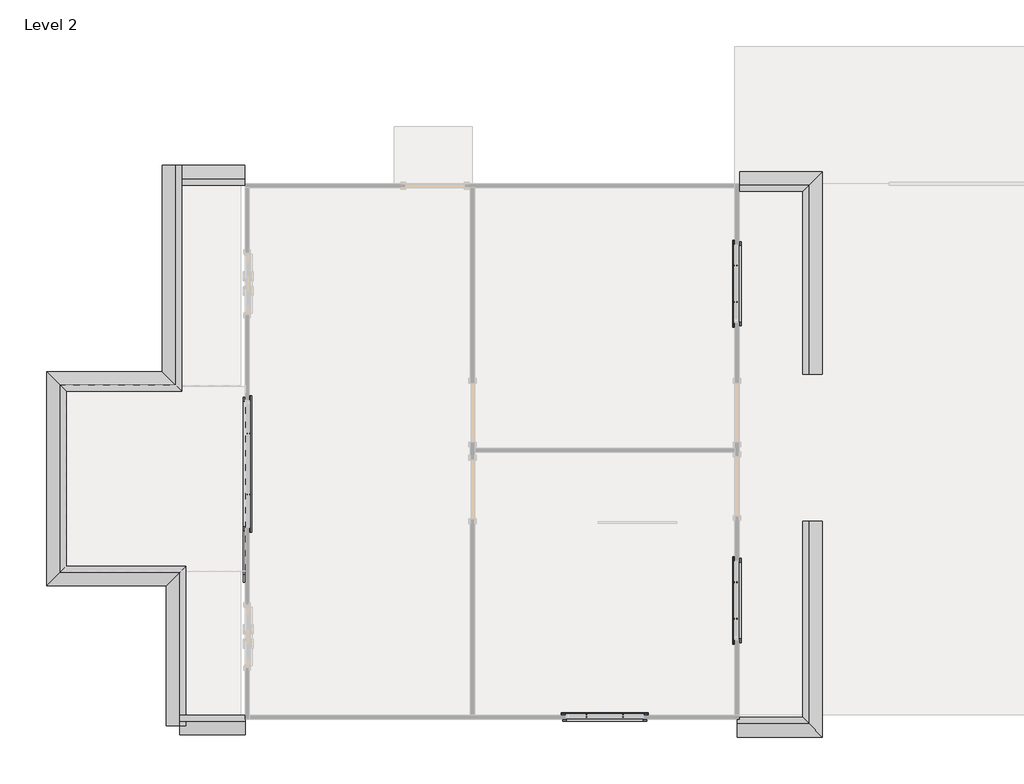
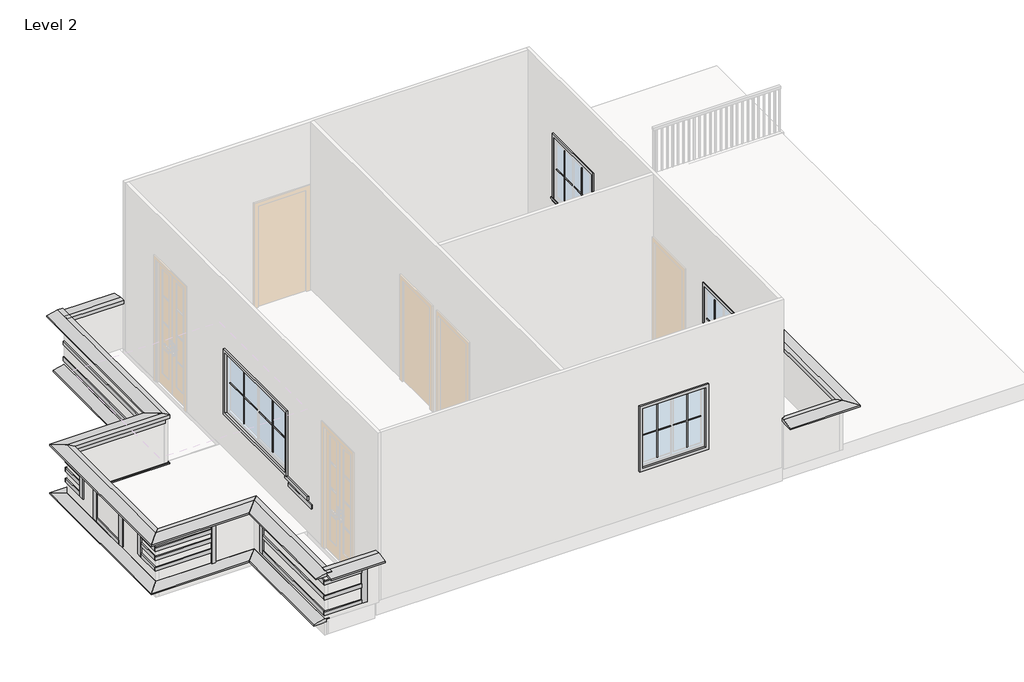
# One storey, part 2 of 2: 41 furniture elements, 34 proxies.
"""IFC4 building model written with IfcOpenShell, lengths in millimetres."""

import ifcopenshell
import ifcopenshell.guid

model = None  # the IFC model being written
_history = None  # IfcOwnerHistory: only IFC2X3 demands one
_inside = {}  # id of a spatial element -> (the spatial element, [elements in it])
_under = {}  # id of a project, library or spatial element -> (it, [spatial elements below it])
_declared = {}  # id of a project -> (the project, [libraries it declares])
_typed = {}  # id of a type object -> (the type object, [elements of that type])
_made_of = {}  # id of a material, layer set ... -> (it, [elements and type objects made of it])


def new_model(schema):
    """Start an empty IFC model of exactly this schema.

    Asked for "IFC4X3", IfcOpenShell would pick the latest addendum, in which some entities
    have other attributes; the version numbers below select the first issue.
    IFC2X3 requires an IfcOwnerHistory on every rooted entity: one is made here for all.
    """
    global model, _history
    if schema == "IFC4X3":
        model = ifcopenshell.file(schema_version=(4, 3, 0, 0))
    else:
        model = ifcopenshell.file(schema=schema)
    _inside.clear()
    _under.clear()
    _declared.clear()
    _typed.clear()
    _made_of.clear()
    _history = None
    if model.schema == "IFC2X3":
        org = make("IfcOrganization", Name="unknown")
        user = make(
            "IfcPersonAndOrganization",
            ThePerson=make("IfcPerson", FamilyName="unknown"),
            TheOrganization=org,
        )
        app = make(
            "IfcApplication",
            ApplicationDeveloper=org,
            Version="unknown",
            ApplicationFullName="unknown",
            ApplicationIdentifier="unknown",
        )
        _history = make(
            "IfcOwnerHistory",
            OwningUser=user,
            OwningApplication=app,
            ChangeAction="ADDED",
            CreationDate=0,
        )
    return model


def make(cls, **values):
    """One entity of the class cls with the attributes given. An attribute that is None is left unset."""
    return model.create_entity(
        cls, **{name: value for name, value in values.items() if value is not None}
    )


def rooted(cls, **values):
    """An entity with a GlobalId (a new one), such as an element, a storey or a relation."""
    return make(cls, GlobalId=ifcopenshell.guid.new(), OwnerHistory=_history, **values)


def si_unit(unit_type, name, prefix=None):
    """IfcSIUnit, for example si_unit("LENGTHUNIT", "METRE", prefix="MILLI")."""
    return make("IfcSIUnit", UnitType=unit_type, Prefix=prefix, Name=name)


def assignment(units):
    """IfcUnitAssignment: the units of a project."""
    return None if units is None else make("IfcUnitAssignment", Units=units)


def point(xyz):
    """IfcCartesianPoint."""
    return None if xyz is None else make("IfcCartesianPoint", Coordinates=xyz)


def direction(xyz):
    """IfcDirection."""
    return None if xyz is None else make("IfcDirection", DirectionRatios=xyz)


def frame(location, z_axis=None, x_axis=None):
    """IfcAxis2Placement3D, a coordinate frame: its origin and axes. An axis left out is left unset."""
    return make(
        "IfcAxis2Placement3D",
        Location=point(location),
        Axis=direction(z_axis),
        RefDirection=direction(x_axis),
    )


def origin():
    """The frame at (0, 0, 0) with its axes left unset."""
    return frame((0.0, 0.0, 0.0))


def origin_with_axes():
    """The frame at (0, 0, 0) with the z axis (0, 0, 1) and the x axis (1, 0, 0) written out."""
    return frame((0.0, 0.0, 0.0), z_axis=(0.0, 0.0, 1.0), x_axis=(1.0, 0.0, 0.0))


def place(relative_to, where):
    """IfcLocalPlacement: puts the frame where relative to a parent placement (None: the world)."""
    return make(
        "IfcLocalPlacement", PlacementRelTo=relative_to, RelativePlacement=where
    )


def context(
    kind, dimensions, precision=None, world=None, true_north=None, identifier=None
):
    """IfcGeometricRepresentationContext, for example the 3D "Model" context."""
    return make(
        "IfcGeometricRepresentationContext",
        ContextIdentifier=identifier,
        ContextType=kind,
        CoordinateSpaceDimension=dimensions,
        Precision=precision,
        WorldCoordinateSystem=world,
        TrueNorth=true_north,
    )


def project(units=None, contexts=None):
    """IfcProject with its units and contexts."""
    return rooted(
        "IfcProject",
        Name="project",
        RepresentationContexts=contexts,
        UnitsInContext=assignment(units),
    )


def spatial(cls, under=None, at=None, **own):
    """A site, building, storey or space (cls), placed at a placement, below another one or the project."""
    s = rooted(cls, ObjectPlacement=at, **own)
    if under is not None:
        _under.setdefault(under.id(), (under, []))[1].append(s)
    return s


def polyline(points):
    """IfcPolyline through the points."""
    return make("IfcPolyline", Points=[point(p) for p in points])


def outline(outer, holes=None, kind="AREA"):
    """IfcArbitraryClosedProfileDef: a profile drawn as a closed curve; with holes, ...WithVoids."""
    if holes is None:
        return make("IfcArbitraryClosedProfileDef", ProfileType=kind, OuterCurve=outer)
    return make(
        "IfcArbitraryProfileDefWithVoids",
        ProfileType=kind,
        OuterCurve=outer,
        InnerCurves=holes,
    )


def extrude(swept, where, along, depth):
    """IfcExtrudedAreaSolid: the profile swept, set in the frame where, extruded along a direction by depth."""
    return make(
        "IfcExtrudedAreaSolid",
        SweptArea=swept,
        Position=where,
        ExtrudedDirection=direction(along),
        Depth=depth,
    )


def faces_of(points, faces, orient=None, outer=None):
    """IfcFace entities. A face is a list of loops; a loop is a list of indices into points, from 0.

    orient and outer hold one flag for each loop. By default every Orientation is true, the
    first loop of a face is its IfcFaceOuterBound and the others are IfcFaceBound.
    """
    made = []
    for i, loops in enumerate(faces):
        bounds = []
        for j, loop in enumerate(loops):
            is_outer = j == 0 if outer is None else outer[i][j]
            bounds.append(
                make(
                    "IfcFaceOuterBound" if is_outer else "IfcFaceBound",
                    Bound=make("IfcPolyLoop", Polygon=[points[k] for k in loop]),
                    Orientation=True if orient is None else orient[i][j],
                )
            )
        made.append(make("IfcFace", Bounds=bounds))
    return made


def faceted_brep(points, faces, orient=None, outer=None, voids=None):
    """IfcFacetedBrep: a solid bounded by flat faces; with voids (closed shells), ...WithVoids."""
    shared = [point(p) for p in points]
    hull = make("IfcClosedShell", CfsFaces=faces_of(shared, faces, orient, outer))
    if voids is None:
        return make("IfcFacetedBrep", Outer=hull)
    return make(
        "IfcFacetedBrepWithVoids",
        Outer=hull,
        Voids=[
            make(cls, CfsFaces=faces_of(shared, fs, o, b)) for cls, fs, o, b in voids
        ],
    )


def shape(context_of_items, identifier, shape_type, items):
    """IfcShapeRepresentation: the items that make up one representation, for example the "Body"."""
    return make(
        "IfcShapeRepresentation",
        ContextOfItems=context_of_items,
        RepresentationIdentifier=identifier,
        RepresentationType=shape_type,
        Items=items,
    )


def source(mapping_origin, context_of_items, identifier, shape_type, items):
    """IfcRepresentationMap: a shape defined once, which mapped items show again and again."""
    return make(
        "IfcRepresentationMap",
        MappingOrigin=mapping_origin,
        MappedRepresentation=shape(context_of_items, identifier, shape_type, items),
    )


def transform(
    local_origin,
    x_axis=None,
    y_axis=None,
    z_axis=None,
    scale=None,
    scale2=None,
    scale3=None,
    uniform=True,
):
    """IfcCartesianTransformationOperator3D, or its non-uniform kind. x_axis, y_axis, z_axis: its Axis1, 2, 3."""
    if uniform:
        return make(
            "IfcCartesianTransformationOperator3D",
            Axis1=direction(x_axis),
            Axis2=direction(y_axis),
            LocalOrigin=point(local_origin),
            Scale=scale,
            Axis3=direction(z_axis),
        )
    return make(
        "IfcCartesianTransformationOperator3DnonUniform",
        Axis1=direction(x_axis),
        Axis2=direction(y_axis),
        LocalOrigin=point(local_origin),
        Scale=scale,
        Axis3=direction(z_axis),
        Scale2=scale2,
        Scale3=scale3,
    )


def mapped(mapping_source, mapping_target):
    """IfcMappedItem: shows the shape of a source again, moved by a transform."""
    return make(
        "IfcMappedItem", MappingSource=mapping_source, MappingTarget=mapping_target
    )


def made_of(thing, what):
    """Note that an element or type object is made of a material, layer set ...; save() writes the relation."""
    if what is not None:
        _made_of.setdefault(what.id(), (what, []))[1].append(thing)
    return thing


def element(
    cls,
    number,
    at=None,
    inside=None,
    cuts=None,
    type_object=None,
    material=None,
    context=None,
    identifier="Body",
    shape_type=None,
    held_by="IfcProductDefinitionShape",
    body=None,
    shapes=None,
    **own,
):
    """One element of the class cls, such as IfcWall. Its Tag is "e" and its number.

    at: its placement. inside: the storey or other place that contains it. cuts: it is an
    opening in that element (IfcRelVoidsElement). A single representation is given by context,
    identifier, shape_type and body (its items); several are given by shapes. held_by: the class
    of the entity that holds the representations. save() writes the other relations.
    """
    e = rooted(cls, Tag="e%d" % number, ObjectPlacement=at, **own)
    if body is not None:
        shapes = [shape(context, identifier, shape_type, body)]
    if shapes is not None:
        e.Representation = make(held_by, Representations=shapes)
    if inside is not None:
        _inside.setdefault(inside.id(), (inside, []))[1].append(e)
    if cuts is not None:
        rooted(
            "IfcRelVoidsElement", RelatingBuildingElement=cuts, RelatedOpeningElement=e
        )
    if type_object is not None:
        _typed.setdefault(type_object.id(), (type_object, []))[1].append(e)
    return made_of(e, material)


def aggregate(whole, parts):
    """IfcRelAggregates: a whole, such as a stair, and the parts it consists of."""
    return rooted("IfcRelAggregates", RelatingObject=whole, RelatedObjects=parts)


def save(model, path):
    """Write the relations noted so far, then the file.

    IfcRelAggregates (storeys below a building ...), IfcRelContainedInSpatialStructure (elements
    in a storey), IfcRelDefinesByType, IfcRelAssociatesMaterial and IfcRelDeclares: one each for
    every whole, place, type object, material and project.
    """
    for whole, parts in _under.values():
        aggregate(whole, parts)
    for where, things in _inside.values():
        rooted(
            "IfcRelContainedInSpatialStructure",
            RelatedElements=things,
            RelatingStructure=where,
        )
    for kind, things in _typed.values():
        rooted("IfcRelDefinesByType", RelatedObjects=things, RelatingType=kind)
    for what, things in _made_of.values():
        rooted("IfcRelAssociatesMaterial", RelatedObjects=things, RelatingMaterial=what)
    for by, libraries in _declared.values():
        rooted("IfcRelDeclares", RelatingContext=by, RelatedDefinitions=libraries)
    model.write(path)


def muntin_pattern_2x2_muntin_pattern_2x2_cf37b409(model_context):
    return source(origin(), model_context, "Body", "SweptSolid", [
        extrude(outline(polyline([(542.925, -6.35), (542.925, -261.9375), (530.225, -261.9375), (530.225, -6.35), (0.0, -6.35), (0.0, 6.35), (530.225, 6.35), (530.225, 261.9375), (542.925, 261.9375), (542.925, 6.35), (1073.15, 6.35), (1073.15, -6.35), (542.925, -6.35)])), frame((0.0, 9.525, 0.0), z_axis=(0.0, 1.0, 0.0), x_axis=(0.0, 0.0, 1.0)), (0.0, 0.0, 1.0), 12.7),
        extrude(outline(polyline([(542.925, -6.35), (542.925, -261.9375), (530.225, -261.9375), (530.225, -6.35), (0.0, -6.35), (0.0, 6.35), (530.225, 6.35), (530.225, 261.9375), (542.925, 261.9375), (542.925, 6.35), (1073.15, 6.35), (1073.15, -6.35), (542.925, -6.35)])), frame((0.0, -22.225, 0.0), z_axis=(0.0, 1.0, 0.0), x_axis=(0.0, 0.0, 1.0)), (0.0, 0.0, 1.0), 12.7),
    ])


def muntin_pattern_2x2_muntin_pattern_2x2_4e1ccfa3(model_context):
    return source(origin(), model_context, "Body", "SweptSolid", [
        extrude(outline(polyline([(542.925, -6.35), (542.925, -452.4375), (530.225, -452.4375), (530.225, -6.35), (0.0, -6.35), (0.0, 6.35), (530.225, 6.35), (530.225, 452.4375), (542.925, 452.4375), (542.925, 6.35), (1073.15, 6.35), (1073.15, -6.35), (542.925, -6.35)])), frame((0.0, 9.525, 0.0), z_axis=(0.0, 1.0, 0.0), x_axis=(0.0, 0.0, 1.0)), (0.0, 0.0, 1.0), 12.7),
        extrude(outline(polyline([(542.925, -6.35), (542.925, -452.4375), (530.225, -452.4375), (530.225, -6.35), (0.0, -6.35), (0.0, 6.35), (530.225, 6.35), (530.225, 452.4375), (542.925, 452.4375), (542.925, 6.35), (1073.15, 6.35), (1073.15, -6.35), (542.925, -6.35)])), frame((0.0, -22.225, 0.0), z_axis=(0.0, 1.0, 0.0), x_axis=(0.0, 0.0, 1.0)), (0.0, 0.0, 1.0), 12.7),
    ])


def trim_window_exterior_flat_with_sill_7cfdd449(model_context):
    return source(origin(), model_context, "Body", "SweptSolid", [
        extrude(outline(polyline([(666.75, -1241.3823709), (666.75, -1298.5323709), (-666.75, -1298.5323709), (-666.75, -1241.3823709), (666.75, -1241.3823709)])), origin_with_axes(), (0.0, 0.0, 1.0), 19.05),
        extrude(outline(polyline([(-1250.95, 38.1), (-1221.6580645, 38.1), (-1219.2, 19.05), (-1219.2, 0.0), (-1241.3823709, 0.0), (-1241.3823709, 19.05), (-1250.95, 19.05), (-1250.95, 38.1)])), frame((-679.45, 0.0, 0.0), z_axis=(1.0, 0.0, 0.0), x_axis=(0.0, 1.0, 0.0)), (0.0, 0.0, 1.0), 1358.9),
        extrude(outline(polyline([(-666.75, 57.15), (666.75, 57.15), (666.75, -1219.2), (609.6, -1219.2), (609.6, 0.0), (-609.6, 0.0), (-609.6, -1219.2), (-666.75, -1219.2), (-666.75, 57.15)])), origin_with_axes(), (0.0, 0.0, 1.0), 19.05),
    ])


def trim_window_exterior_flat_with_sill_97a7de1c(model_context):
    return source(origin(), model_context, "Body", "SweptSolid", [
        extrude(outline(polyline([(1047.75, -1241.3823709), (1047.75, -1298.5323709), (-1047.75, -1298.5323709), (-1047.75, -1241.3823709), (1047.75, -1241.3823709)])), origin_with_axes(), (0.0, 0.0, 1.0), 19.05),
        extrude(outline(polyline([(-1250.95, 38.1), (-1221.6580645, 38.1), (-1219.2, 19.05), (-1219.2, 0.0), (-1241.3823709, 0.0), (-1241.3823709, 19.05), (-1250.95, 19.05), (-1250.95, 38.1)])), frame((-1060.45, 0.0, 0.0), z_axis=(1.0, 0.0, 0.0), x_axis=(0.0, 1.0, 0.0)), (0.0, 0.0, 1.0), 2120.9),
        extrude(outline(polyline([(-1047.75, 57.15), (1047.75, 57.15), (1047.75, -1219.2), (990.6, -1219.2), (990.6, 0.0), (-990.6, 0.0), (-990.6, -1219.2), (-1047.75, -1219.2), (-1047.75, 57.15)])), origin_with_axes(), (0.0, 0.0, 1.0), 19.05),
    ])


def trim_window_interior_flat_picture_frame_f1e0b15b(model_context):
    return source(origin(), model_context, "Body", "SweptSolid", [
        extrude(outline(polyline([(654.05, 44.45), (654.05, -1263.65), (-654.05, -1263.65), (-654.05, 44.45), (654.05, 44.45)]), holes=[polyline([(596.9, -12.7), (-596.9, -12.7), (-596.9, -1206.5), (596.9, -1206.5), (596.9, -12.7)])]), origin_with_axes(), (0.0, 0.0, 1.0), 31.75),
    ])


def trim_window_interior_flat_picture_frame_b9d4c0b4(model_context):
    return source(origin(), model_context, "Body", "SweptSolid", [
        extrude(outline(polyline([(1035.05, 44.45), (1035.05, -1263.65), (-1035.05, -1263.65), (-1035.05, 44.45), (1035.05, 44.45)]), holes=[polyline([(977.9, -12.7), (-977.9, -12.7), (-977.9, -1206.5), (977.9, -1206.5), (977.9, -12.7)])]), origin_with_axes(), (0.0, 0.0, 1.0), 31.75),
    ])


def m_upper_cabinet_filler_wall_65b3d82e(model_context):
    return source(origin(), model_context, "Body", "SweptSolid", [
        extrude(outline(polyline([(-198.8288372, 38.1), (-198.8288372, 57.15), (258.3711628, 57.15), (258.3711628, 38.1), (-198.8288372, 38.1)])), frame((0.0, 0.0, 1923.8), z_axis=(0.0, 0.0, 1.0), x_axis=(1.0, 0.0, 0.0)), (0.0, 0.0, 1.0), 76.2),
    ])


def m_upper_cabinet_filler_wall_c56b41ac(model_context):
    return source(origin(), model_context, "Body", "SweptSolid", [
        extrude(outline(polyline([(-21.0288372, 38.1), (-21.0288372, 57.15), (80.5711628, 57.15), (80.5711628, 38.1), (-21.0288372, 38.1)])), frame((0.0, 0.0, 1531.6875), z_axis=(0.0, 0.0, 1.0), x_axis=(1.0, 0.0, 0.0)), (0.0, 0.0, 1.0), 468.3125),
    ])


def m_upper_cabinet_filler_wall_ea785238(model_context):
    return source(origin(), model_context, "Body", "SweptSolid", [
        extrude(outline(polyline([(-503.6288372, 38.1), (-503.6288372, 57.15), (563.1711628, 57.15), (563.1711628, 38.1), (-503.6288372, 38.1)])), frame((0.0, 0.0, 1923.8), z_axis=(0.0, 0.0, 1.0), x_axis=(1.0, 0.0, 0.0)), (0.0, 0.0, 1.0), 76.2),
    ])


def m_upper_cabinet_filler_wall_177953ad(model_context):
    return source(origin(), model_context, "Body", "SweptSolid", [
        extrude(outline(polyline([(-8.3288372, 38.1), (-8.3288372, 57.15), (67.8711628, 57.15), (67.8711628, 38.1), (-8.3288372, 38.1)])), frame((0.0, 0.0, 1085.6), z_axis=(0.0, 0.0, 1.0), x_axis=(1.0, 0.0, 0.0)), (0.0, 0.0, 1.0), 914.4),
    ])


def m_upper_cabinet_filler_wall_75mm_90d919fc(model_context):
    return source(origin(), model_context, "Body", "SweptSolid", [
        extrude(outline(polyline([(-21.0288372, 38.1), (-21.0288372, 57.15), (80.5711628, 57.15), (80.5711628, 38.1), (-21.0288372, 38.1)])), frame((0.0, 0.0, 1314.2), z_axis=(0.0, 0.0, 1.0), x_axis=(1.0, 0.0, 0.0)), (0.0, 0.0, 1.0), 685.8),
    ])


def m_upper_cabinet_filler_wall_75mm_2_2fb8ce97(model_context):
    return source(origin(), model_context, "Body", "SweptSolid", [
        extrude(outline(polyline([(-21.0288372, 88.9), (-21.0288372, 107.95), (80.5711628, 107.95), (80.5711628, 88.9), (-21.0288372, 88.9)])), frame((0.0, 0.0, 1314.1523437), z_axis=(0.0, 0.0, 1.0), x_axis=(1.0, 0.0, 0.0)), (0.0, 0.0, 1.0), 685.8),
    ])


def m_upper_cabinet_filler_wall_horizontal_0d8bff8c(model_context):
    return source(origin(), model_context, "Body", "SweptSolid", [
        extrude(outline(polyline([(-325.8288372, 38.1), (-325.8288372, 57.15), (385.3711628, 57.15), (385.3711628, 38.1), (-325.8288372, 38.1)])), frame((0.0, 0.0, 1923.8), z_axis=(0.0, 0.0, 1.0), x_axis=(1.0, 0.0, 0.0)), (0.0, 0.0, 1.0), 76.2),
    ])


def m_upper_cabinet_filler_wall_horizontal_2_28a204f3(model_context):
    return source(origin(), model_context, "Body", "SweptSolid", [
        extrude(outline(polyline([(-344.8788372, 38.1), (-344.8788372, 57.15), (404.4211628, 57.15), (404.4211628, 38.1), (-344.8788372, 38.1)])), frame((0.0, 0.0, 1923.8), z_axis=(0.0, 0.0, 1.0), x_axis=(1.0, 0.0, 0.0)), (0.0, 0.0, 1.0), 76.2),
    ])


def m_upper_cabinet_filler_wall_horizontal_3_602a78bd(model_context):
    return source(origin(), model_context, "Body", "SweptSolid", [
        extrude(outline(polyline([(-967.1788372, 38.1), (-967.1788372, 57.15), (1026.7211628, 57.15), (1026.7211628, 38.1), (-967.1788372, 38.1)])), frame((0.0, 0.0, 1923.8), z_axis=(0.0, 0.0, 1.0), x_axis=(1.0, 0.0, 0.0)), (0.0, 0.0, 1.0), 76.2),
    ])


def m_upper_cabinet_filler_wall_horizontal_4_0c22a44f(model_context):
    return source(origin(), model_context, "Body", "SweptSolid", [
        extrude(outline(polyline([(-1411.6788372, 38.1), (-1411.6788372, 57.15), (1471.2211628, 57.15), (1471.2211628, 38.1), (-1411.6788372, 38.1)])), frame((0.0, 0.0, 1923.8), z_axis=(0.0, 0.0, 1.0), x_axis=(1.0, 0.0, 0.0)), (0.0, 0.0, 1.0), 76.2),
    ])


def m_upper_cabinet_filler_wall_horizontal_5_76bebc23(model_context):
    return source(origin(), model_context, "Body", "SweptSolid", [
        extrude(outline(polyline([(-344.8788372, 88.9), (-344.8788372, 107.95), (404.4211628, 107.95), (404.4211628, 88.9), (-344.8788372, 88.9)])), frame((0.0, 0.0, 1923.8), z_axis=(0.0, 0.0, 1.0), x_axis=(1.0, 0.0, 0.0)), (0.0, 0.0, 1.0), 76.2),
    ])


model = new_model("IFC4")

# Units and contexts
model_context = context("Model", 3, world=origin())
ifc_project = project(units=[si_unit("LENGTHUNIT", "METRE", prefix="MILLI")], contexts=[model_context])

# Site, building, storey
site = spatial("IfcSite", under=ifc_project)
building = spatial("IfcBuilding", under=site)
storey = spatial("IfcBuildingStorey", under=building, Name="Level 2", Elevation=3352.8)

# Proxies
placement = place(None, origin())
element("IfcBuildingElementProxy", 1, Name="Cornice", ObjectType="Cornice", at=placement, inside=storey, context=model_context, shape_type="Brep", body=[
    faceted_brep([(194.9904617, 1366.1708836, 4337.05), (194.9904617, 1366.1708836, 4267.2), (499.7904617, 1061.3708836, 4267.2), (499.7904617, 1061.3708836, 4292.6), (287.0654617, 1274.0958836, 4337.05), (194.9904617, 4414.6042394, 4337.05), (287.0654617, 4414.6042394, 4337.05), (499.7904617, 4414.6042394, 4292.6), (499.7904617, 4414.6042394, 4267.2), (194.9904617, 4414.6042394, 4267.2)], [[[0, 1, 2, 3, 4]], [[5, 6, 7, 8, 9]], [[2, 1, 9, 8]], [[3, 2, 8, 7]], [[0, 4, 6, 5]], [[1, 0, 5, 9]], [[4, 3, 7, 6]]]),
    faceted_brep([(194.9904617, 6700.6042394, 4337.05), (194.9904617, 6700.6042394, 4267.2), (499.7904617, 6700.6042394, 4267.2), (499.7904617, 6700.6042394, 4292.6), (287.0654617, 6700.6042394, 4337.05), (194.9904617, 9551.3208836, 4337.05), (287.0654617, 9643.3958836, 4337.05), (499.7904617, 9856.1208836, 4292.6), (499.7904617, 9856.1208836, 4267.2), (194.9904617, 9551.3208836, 4267.2)], [[[0, 1, 2, 3, 4]], [[5, 6, 7, 8, 9]], [[2, 1, 9, 8]], [[3, 2, 8, 7]], [[0, 4, 6, 5]], [[1, 0, 5, 9]], [[4, 3, 7, 6]]]),
])
element("IfcBuildingElementProxy", 2, Name="Cornice", ObjectType="Cornice", at=placement, inside=storey, context=model_context, shape_type="Brep", body=[
    faceted_brep([(194.9904617, 1366.1708836, 4337.05), (287.0654617, 1274.0958836, 4337.05), (499.7904617, 1061.3708836, 4292.6), (499.7904617, 1061.3708836, 4267.2), (194.9904617, 1366.1708836, 4267.2), (-827.1648468, 1366.1708836, 4337.05), (-827.1648468, 1366.1708836, 4267.2), (-827.1648468, 1061.3708836, 4267.2), (-827.1648468, 1061.3708836, 4292.6), (-827.1648468, 1274.0958836, 4337.05)], [[[0, 1, 2, 3, 4]], [[5, 6, 7, 8, 9]], [[0, 4, 6, 5]], [[1, 0, 5, 9]], [[3, 2, 8, 7]], [[4, 3, 7, 6]], [[2, 1, 9, 8]]]),
])
element("IfcBuildingElementProxy", 3, Name="Cornice", ObjectType="Cornice", at=placement, inside=storey, context=model_context, shape_type="Brep", body=[
    faceted_brep([(194.9904617, 9551.3208836, 4337.05), (194.9904617, 9551.3208836, 4267.2), (499.7904617, 9856.1208836, 4267.2), (499.7904617, 9856.1208836, 4292.6), (287.0654617, 9643.3958836, 4337.05), (-786.0845383, 9551.3208836, 4337.05), (-786.0845383, 9643.3958836, 4337.05), (-786.0845383, 9856.1208836, 4292.6), (-786.0845383, 9856.1208836, 4267.2), (-786.0845383, 9551.3208836, 4267.2)], [[[0, 1, 2, 3, 4]], [[5, 6, 7, 8, 9]], [[2, 1, 9, 8]], [[3, 2, 8, 7]], [[0, 4, 6, 5]], [[1, 0, 5, 9]], [[4, 3, 7, 6]]]),
])
element("IfcBuildingElementProxy", 4, Name="Cornice", ObjectType="Cornice", at=placement, inside=storey, context=model_context, shape_type="SweptSolid", body=[
    extrude(outline(polyline([(9648.1405032, 4337.05), (9740.2155032, 4337.05), (9952.9405032, 4292.6), (9952.9405032, 4267.2), (9648.1405032, 4267.2), (9648.1405032, 4337.05)])), frame((-9558.0643703, 0.0, 0.0), z_axis=(1.0, 0.0, 0.0), x_axis=(0.0, 1.0, 0.0)), (0.0, 0.0, 1.0), 1073.15),
])
element("IfcBuildingElementProxy", 5, Name="Cornice", ObjectType="Cornice", at=placement, inside=storey, context=model_context, shape_type="Brep", body=[
    faceted_brep([(-9465.9893703, 9952.9405032, 4337.05), (-9465.9893703, 9952.9405032, 4267.2), (-9770.7893703, 9952.9405032, 4267.2), (-9770.7893703, 9952.9405032, 4292.6), (-9558.0643703, 9952.9405032, 4337.05), (-9465.9893703, 6437.6391758, 4337.05), (-9558.0643703, 6529.7141758, 4337.05), (-9770.7893703, 6742.4391758, 4292.6), (-9770.7893703, 6742.4391758, 4267.2), (-9465.9893703, 6437.6391758, 4267.2)], [[[0, 1, 2, 3, 4]], [[5, 6, 7, 8, 9]], [[2, 1, 9, 8]], [[3, 2, 8, 7]], [[0, 4, 6, 5]], [[1, 0, 5, 9]], [[4, 3, 7, 6]]]),
])
element("IfcBuildingElementProxy", 6, Name="Cornice", ObjectType="Cornice", at=placement, inside=storey, context=model_context, shape_type="Brep", body=[
    faceted_brep([(-9465.9893703, 6437.6391758, 4337.05), (-9465.9893703, 6437.6391758, 4267.2), (-9770.7893703, 6742.4391758, 4267.2), (-9770.7893703, 6742.4391758, 4292.6), (-9558.0643703, 6529.7141758, 4337.05), (-11263.0393703, 6437.6391758, 4337.05), (-11355.1143703, 6529.7141758, 4337.05), (-11567.8393703, 6742.4391758, 4292.6), (-11567.8393703, 6742.4391758, 4267.2), (-11263.0393703, 6437.6391758, 4267.2)], [[[0, 1, 2, 3, 4]], [[5, 6, 7, 8, 9]], [[2, 1, 9, 8]], [[3, 2, 8, 7]], [[0, 4, 6, 5]], [[1, 0, 5, 9]], [[4, 3, 7, 6]]]),
])
element("IfcBuildingElementProxy", 7, Name="Cornice", ObjectType="Cornice", at=placement, inside=storey, context=model_context, shape_type="Brep", body=[
    faceted_brep([(-11263.0393703, 6437.6391758, 4337.05), (-11263.0393703, 6437.6391758, 4267.2), (-11567.8393703, 6742.4391758, 4267.2), (-11567.8393703, 6742.4391758, 4292.6), (-11355.1143703, 6529.7141758, 4337.05), (-11263.0393703, 3715.6708836, 4337.05), (-11355.1143703, 3623.5958836, 4337.05), (-11567.8393703, 3410.8708836, 4292.6), (-11567.8393703, 3410.8708836, 4267.2), (-11263.0393703, 3715.6708836, 4267.2)], [[[0, 1, 2, 3, 4]], [[5, 6, 7, 8, 9]], [[2, 1, 9, 8]], [[3, 2, 8, 7]], [[0, 4, 6, 5]], [[1, 0, 5, 9]], [[4, 3, 7, 6]]]),
])
element("IfcBuildingElementProxy", 8, Name="Cornice", ObjectType="Cornice", at=placement, inside=storey, context=model_context, shape_type="SweptSolid", body=[
    extrude(outline(polyline([(1397.9208836, 4337.05), (1397.9208836, 4267.2), (1093.1208836, 4267.2), (1093.1208836, 4292.6), (1305.8458836, 4337.05), (1397.9208836, 4337.05)])), frame((-9494.9148468, 0.0, 0.0), z_axis=(1.0, 0.0, 0.0), x_axis=(0.0, 1.0, 0.0)), (0.0, 0.0, 1.0), 1016.0),
])
element("IfcBuildingElementProxy", 9, Name="Cornice", ObjectType="Cornice", at=placement, inside=storey, context=model_context, shape_type="Brep", body=[
    faceted_brep([(-9402.8398468, 3715.6708836, 4337.05), (-9402.8398468, 3715.6708836, 4267.2), (-9707.6398468, 3410.8708836, 4267.2), (-9707.6398468, 3410.8708836, 4292.6), (-9494.9148468, 3623.5958836, 4337.05), (-9402.8398468, 1235.9958836, 4337.05), (-9494.9148468, 1235.9958836, 4337.05), (-9707.6398468, 1235.9958836, 4292.6), (-9707.6398468, 1235.9958836, 4267.2), (-9402.8398468, 1235.9958836, 4267.2)], [[[0, 1, 2, 3, 4]], [[5, 6, 7, 8, 9]], [[2, 1, 9, 8]], [[3, 2, 8, 7]], [[0, 4, 6, 5]], [[1, 0, 5, 9]], [[4, 3, 7, 6]]]),
])
element("IfcBuildingElementProxy", 10, Name="Cornice", ObjectType="Cornice", at=placement, inside=storey, context=model_context, shape_type="Brep", body=[
    faceted_brep([(-11263.0393703, 3715.6708836, 4337.05), (-11263.0393703, 3715.6708836, 4267.2), (-11567.8393703, 3410.8708836, 4267.2), (-11567.8393703, 3410.8708836, 4292.6), (-11355.1143703, 3623.5958836, 4337.05), (-9402.8398468, 3715.6708836, 4337.05), (-9494.9148468, 3623.5958836, 4337.05), (-9707.6398468, 3410.8708836, 4292.6), (-9707.6398468, 3410.8708836, 4267.2), (-9402.8398468, 3715.6708836, 4267.2)], [[[0, 1, 2, 3, 4]], [[5, 6, 7, 8, 9]], [[2, 1, 9, 8]], [[3, 2, 8, 7]], [[0, 4, 6, 5]], [[1, 0, 5, 9]], [[4, 3, 7, 6]]]),
])
element("IfcBuildingElementProxy", 11, Name="Cornice", ObjectType="Cornice", at=placement, inside=storey, context=model_context, shape_type="Brep", body=[
    faceted_brep([(-9465.9893703, 9740.2155032, 3371.85), (-9465.9893703, 9740.2155032, 3302.0), (-9770.7893703, 9740.2155032, 3302.0), (-9770.7893703, 9740.2155032, 3327.4), (-9558.0643703, 9740.2155032, 3371.85), (-9465.9893703, 6437.6391758, 3371.85), (-9558.0643703, 6529.7141758, 3371.85), (-9770.7893703, 6742.4391758, 3327.4), (-9770.7893703, 6742.4391758, 3302.0), (-9465.9893703, 6437.6391758, 3302.0)], [[[0, 1, 2, 3, 4]], [[5, 6, 7, 8, 9]], [[1, 0, 5, 9]], [[2, 1, 9, 8]], [[3, 2, 8, 7]], [[4, 3, 7, 6]], [[0, 4, 6, 5]]]),
])
element("IfcBuildingElementProxy", 12, Name="Cornice 3", ObjectType="Cornice 3", at=placement, inside=storey, context=model_context, shape_type="Brep", body=[
    faceted_brep([(-9402.8398468, 3715.6708836, 3371.85), (-9402.8398468, 3715.6708836, 3302.0), (-9707.6398468, 3410.8708836, 3302.0), (-9707.6398468, 3410.8708836, 3327.4), (-9494.9148468, 3623.5958836, 3371.85), (-9402.8398468, 1305.8458836, 3371.85), (-9494.9148468, 1305.8458836, 3371.85), (-9707.6398468, 1305.8458836, 3327.4), (-9707.6398468, 1305.8458836, 3302.0), (-9402.8398468, 1305.8458836, 3302.0)], [[[0, 1, 2, 3, 4]], [[5, 6, 7, 8, 9]], [[1, 0, 5, 9]], [[2, 1, 9, 8]], [[3, 2, 8, 7]], [[4, 3, 7, 6]], [[0, 4, 6, 5]]]),
])
element("IfcBuildingElementProxy", 13, Name="Cornice 3", ObjectType="Cornice 3", at=placement, inside=storey, context=model_context, shape_type="Brep", body=[
    faceted_brep([(-11263.0393703, 3715.6708836, 3371.85), (-11263.0393703, 3715.6708836, 3302.0), (-11567.8393703, 3410.8708836, 3302.0), (-11567.8393703, 3410.8708836, 3327.4), (-11355.1143703, 3623.5958836, 3371.85), (-9402.8398468, 3715.6708836, 3371.85), (-9494.9148468, 3623.5958836, 3371.85), (-9707.6398468, 3410.8708836, 3327.4), (-9707.6398468, 3410.8708836, 3302.0), (-9402.8398468, 3715.6708836, 3302.0)], [[[0, 1, 2, 3, 4]], [[5, 6, 7, 8, 9]], [[1, 0, 5, 9]], [[2, 1, 9, 8]], [[3, 2, 8, 7]], [[4, 3, 7, 6]], [[0, 4, 6, 5]]]),
])
element("IfcBuildingElementProxy", 14, Name="Cornice 3", ObjectType="Cornice 3", at=placement, inside=storey, context=model_context, shape_type="Brep", body=[
    faceted_brep([(-11263.0393703, 6437.6391758, 3371.85), (-11263.0393703, 6437.6391758, 3302.0), (-11567.8393703, 6742.4391758, 3302.0), (-11567.8393703, 6742.4391758, 3327.4), (-11355.1143703, 6529.7141758, 3371.85), (-11263.0393703, 3715.6708836, 3371.85), (-11355.1143703, 3623.5958836, 3371.85), (-11567.8393703, 3410.8708836, 3327.4), (-11567.8393703, 3410.8708836, 3302.0), (-11263.0393703, 3715.6708836, 3302.0)], [[[0, 1, 2, 3, 4]], [[5, 6, 7, 8, 9]], [[1, 0, 5, 9]], [[2, 1, 9, 8]], [[3, 2, 8, 7]], [[4, 3, 7, 6]], [[0, 4, 6, 5]]]),
])
element("IfcBuildingElementProxy", 15, Name="Cornice 3", ObjectType="Cornice 3", at=placement, inside=storey, context=model_context, shape_type="Brep", body=[
    faceted_brep([(-9465.9893703, 6437.6391758, 3371.85), (-9465.9893703, 6437.6391758, 3302.0), (-9770.7893703, 6742.4391758, 3302.0), (-9770.7893703, 6742.4391758, 3327.4), (-9558.0643703, 6529.7141758, 3371.85), (-11263.0393703, 6437.6391758, 3371.85), (-11355.1143703, 6529.7141758, 3371.85), (-11567.8393703, 6742.4391758, 3327.4), (-11567.8393703, 6742.4391758, 3302.0), (-11263.0393703, 6437.6391758, 3302.0)], [[[0, 1, 2, 3, 4]], [[5, 6, 7, 8, 9]], [[1, 0, 5, 9]], [[2, 1, 9, 8]], [[3, 2, 8, 7]], [[4, 3, 7, 6]], [[0, 4, 6, 5]]]),
])
element("IfcBuildingElementProxy", 16, Name="Cornice 4", ObjectType="Cornice 4", at=placement, inside=storey, context=model_context, shape_type="SweptSolid", body=[
    extrude(outline(polyline([(4260.85, -11263.0393703), (4260.85, -11355.1143703), (4216.4, -11390.0393703), (4191.0, -11390.0393703), (4191.0, -11263.0393703), (4260.85, -11263.0393703)])), frame((0.0, 3623.5958836, 0.0), z_axis=(0.0, 1.0, 0.0), x_axis=(0.0, 0.0, 1.0)), (0.0, 0.0, 1.0), 2906.1182923),
])
element("IfcBuildingElementProxy", 17, Name="Cornice 4", ObjectType="Cornice 4", at=placement, inside=storey, context=model_context, shape_type="Brep", body=[
    faceted_brep([(-11263.0393703, 3715.6708836, 4260.85), (-11263.0393703, 3715.6708836, 4191.0), (-11390.0393703, 3588.6708836, 4191.0), (-11390.0393703, 3588.6708836, 4216.4), (-11355.1143703, 3623.5958836, 4260.85), (-9494.9148468, 3715.6708836, 4260.85), (-9494.9148468, 3623.5958836, 4260.85), (-9494.9148468, 3588.6708836, 4216.4), (-9494.9148468, 3588.6708836, 4191.0), (-9494.9148468, 3715.6708836, 4191.0)], [[[0, 1, 2, 3, 4]], [[5, 6, 7, 8, 9]], [[1, 0, 5, 9]], [[2, 1, 9, 8]], [[3, 2, 8, 7]], [[4, 3, 7, 6]], [[0, 4, 6, 5]]]),
])
element("IfcBuildingElementProxy", 18, Name="Cornice 4", ObjectType="Cornice 4", at=placement, inside=storey, context=model_context, shape_type="Brep", body=[
    faceted_brep([(-9558.0643703, 6437.6391758, 4260.85), (-9558.0643703, 6437.6391758, 4191.0), (-9558.0643703, 6564.6391758, 4191.0), (-9558.0643703, 6564.6391758, 4216.4), (-9558.0643703, 6529.7141758, 4260.85), (-11263.0393703, 6437.6391758, 4260.85), (-11355.1143703, 6529.7141758, 4260.85), (-11390.0393703, 6564.6391758, 4216.4), (-11390.0393703, 6564.6391758, 4191.0), (-11263.0393703, 6437.6391758, 4191.0)], [[[0, 1, 2, 3, 4]], [[5, 6, 7, 8, 9]], [[1, 0, 5, 9]], [[2, 1, 9, 8]], [[3, 2, 8, 7]], [[4, 3, 7, 6]], [[0, 4, 6, 5]]]),
])
muntin_pattern_2x2_muntin_pattern_2x2_shape = muntin_pattern_2x2_muntin_pattern_2x2_cf37b409(model_context)
element("IfcBuildingElementProxy", 19, Name="Muntin Pattern_2x2 : Muntin Pattern_2x2", ObjectType="Muntin Pattern_2x2 : Muntin Pattern_2x2", at=placement, inside=storey, context=model_context, shape_type="MappedRepresentation", body=[
    mapped(muntin_pattern_2x2_muntin_pattern_2x2_shape, transform((-2600.4023468, 1391.5708836, 4349.75), x_axis=(1.0, 0.0, 0.0), y_axis=(0.0, 1.0, 0.0), z_axis=(0.0, 0.0, 1.0))),
])
element("IfcBuildingElementProxy", 20, Name="Muntin Pattern_2x2 : Muntin Pattern_2x2", ObjectType="Muntin Pattern_2x2 : Muntin Pattern_2x2", at=placement, inside=storey, context=model_context, shape_type="MappedRepresentation", body=[
    mapped(muntin_pattern_2x2_muntin_pattern_2x2_shape, transform((-3168.7273468, 1391.5708836, 4349.75), x_axis=(1.0, 0.0, 0.0), y_axis=(0.0, 1.0, 0.0), z_axis=(0.0, 0.0, 1.0))),
])
element("IfcBuildingElementProxy", 21, Name="Muntin Pattern_2x2 : Muntin Pattern_2x2", ObjectType="Muntin Pattern_2x2 : Muntin Pattern_2x2", at=placement, inside=storey, context=model_context, shape_type="MappedRepresentation", body=[
    mapped(muntin_pattern_2x2_muntin_pattern_2x2_shape, transform((-849.3898468, 8397.2083836, 4349.75), x_axis=(0.0, 1.0, 0.0), y_axis=(-1.0, 0.0, 0.0), z_axis=(0.0, 0.0, 1.0))),
])
element("IfcBuildingElementProxy", 22, Name="Muntin Pattern_2x2 : Muntin Pattern_2x2", ObjectType="Muntin Pattern_2x2 : Muntin Pattern_2x2", at=placement, inside=storey, context=model_context, shape_type="MappedRepresentation", body=[
    mapped(muntin_pattern_2x2_muntin_pattern_2x2_shape, transform((-849.3898468, 7828.8833836, 4349.75), x_axis=(0.0, 1.0, 0.0), y_axis=(-1.0, 0.0, 0.0), z_axis=(0.0, 0.0, 1.0))),
])
element("IfcBuildingElementProxy", 23, Name="Muntin Pattern_2x2 : Muntin Pattern_2x2", ObjectType="Muntin Pattern_2x2 : Muntin Pattern_2x2", at=placement, inside=storey, context=model_context, shape_type="MappedRepresentation", body=[
    mapped(muntin_pattern_2x2_muntin_pattern_2x2_shape, transform((-849.3898468, 3469.6083836, 4349.75), x_axis=(0.0, 1.0, 0.0), y_axis=(-1.0, 0.0, 0.0), z_axis=(0.0, 0.0, 1.0))),
])
element("IfcBuildingElementProxy", 24, Name="Muntin Pattern_2x2 : Muntin Pattern_2x2", ObjectType="Muntin Pattern_2x2 : Muntin Pattern_2x2", at=placement, inside=storey, context=model_context, shape_type="MappedRepresentation", body=[
    mapped(muntin_pattern_2x2_muntin_pattern_2x2_shape, transform((-849.3898468, 2901.2833836, 4349.75), x_axis=(0.0, 1.0, 0.0), y_axis=(-1.0, 0.0, 0.0), z_axis=(0.0, 0.0, 1.0))),
])
muntin_pattern_2x2_muntin_pattern_2x2_2_shape = muntin_pattern_2x2_muntin_pattern_2x2_4e1ccfa3(model_context)
element("IfcBuildingElementProxy", 25, Name="Muntin Pattern_2x2 : Muntin Pattern_2x2", ObjectType="Muntin Pattern_2x2 : Muntin Pattern_2x2", at=placement, inside=storey, context=model_context, shape_type="MappedRepresentation", body=[
    mapped(muntin_pattern_2x2_muntin_pattern_2x2_2_shape, transform((-8424.9398468, 4833.3110922, 4197.35), x_axis=(0.0, -1.0, 0.0), y_axis=(1.0, 0.0, 0.0), z_axis=(0.0, 0.0, 1.0))),
])
element("IfcBuildingElementProxy", 26, Name="Muntin Pattern_2x2 : Muntin Pattern_2x2", ObjectType="Muntin Pattern_2x2 : Muntin Pattern_2x2", at=placement, inside=storey, context=model_context, shape_type="MappedRepresentation", body=[
    mapped(muntin_pattern_2x2_muntin_pattern_2x2_2_shape, transform((-8424.9398468, 5782.6360922, 4197.35), x_axis=(0.0, -1.0, 0.0), y_axis=(1.0, 0.0, 0.0), z_axis=(0.0, 0.0, 1.0))),
])
trim_window_exterior_flat_with_sill_shape = trim_window_exterior_flat_with_sill_7cfdd449(model_context)
element("IfcBuildingElementProxy", 27, Name="Trim-Window-Exterior-Flat : with Sill", ObjectType="Trim-Window-Exterior-Flat : with Sill", at=placement, inside=storey, context=model_context, shape_type="MappedRepresentation", body=[
    mapped(trim_window_exterior_flat_with_sill_shape, transform((-2884.5648468, 1401.0958836, 5486.4), x_axis=(-1.0, 0.0, 0.0), y_axis=(0.0, 0.0, 1.0), z_axis=(0.0, 1.0, 0.0))),
])
element("IfcBuildingElementProxy", 28, Name="Trim-Window-Exterior-Flat : with Sill", ObjectType="Trim-Window-Exterior-Flat : with Sill", at=placement, inside=storey, context=model_context, shape_type="MappedRepresentation", body=[
    mapped(trim_window_exterior_flat_with_sill_shape, transform((-858.9148468, 8113.0458836, 5486.4), x_axis=(0.0, -1.0, 0.0), y_axis=(0.0, 0.0, 1.0), z_axis=(-1.0, 0.0, 0.0))),
])
element("IfcBuildingElementProxy", 29, Name="Trim-Window-Exterior-Flat : with Sill", ObjectType="Trim-Window-Exterior-Flat : with Sill", at=placement, inside=storey, context=model_context, shape_type="MappedRepresentation", body=[
    mapped(trim_window_exterior_flat_with_sill_shape, transform((-858.9148468, 3185.4458836, 5486.4), x_axis=(0.0, -1.0, 0.0), y_axis=(0.0, 0.0, 1.0), z_axis=(-1.0, 0.0, 0.0))),
])
trim_window_exterior_flat_with_sill_2_shape = trim_window_exterior_flat_with_sill_97a7de1c(model_context)
element("IfcBuildingElementProxy", 30, Name="Trim-Window-Exterior-Flat : with Sill", ObjectType="Trim-Window-Exterior-Flat : with Sill", at=placement, inside=storey, context=model_context, shape_type="MappedRepresentation", body=[
    mapped(trim_window_exterior_flat_with_sill_2_shape, transform((-8415.4148468, 5307.9735922, 5334.0), x_axis=(0.0, 1.0, 0.0), y_axis=(0.0, 0.0, 1.0), z_axis=(1.0, 0.0, 0.0))),
])
trim_window_interior_flat_picture_frame_shape = trim_window_interior_flat_picture_frame_f1e0b15b(model_context)
element("IfcBuildingElementProxy", 31, Name="Trim-Window-Interior-Flat : Picture Frame", ObjectType="Trim-Window-Interior-Flat : Picture Frame", at=placement, inside=storey, context=model_context, shape_type="MappedRepresentation", body=[
    mapped(trim_window_interior_flat_picture_frame_shape, transform((-2884.5648468, 1337.5958836, 5486.4), x_axis=(1.0, 0.0, 0.0), y_axis=(0.0, 0.0, 1.0), z_axis=(0.0, -1.0, 0.0))),
])
element("IfcBuildingElementProxy", 32, Name="Trim-Window-Interior-Flat : Picture Frame", ObjectType="Trim-Window-Interior-Flat : Picture Frame", at=placement, inside=storey, context=model_context, shape_type="MappedRepresentation", body=[
    mapped(trim_window_interior_flat_picture_frame_shape, transform((-795.4148468, 8113.0458836, 5486.4), x_axis=(0.0, 1.0, 0.0), y_axis=(0.0, 0.0, 1.0), z_axis=(1.0, 0.0, 0.0))),
])
element("IfcBuildingElementProxy", 33, Name="Trim-Window-Interior-Flat : Picture Frame", ObjectType="Trim-Window-Interior-Flat : Picture Frame", at=placement, inside=storey, context=model_context, shape_type="MappedRepresentation", body=[
    mapped(trim_window_interior_flat_picture_frame_shape, transform((-795.4148468, 3185.4458836, 5486.4), x_axis=(0.0, 1.0, 0.0), y_axis=(0.0, 0.0, 1.0), z_axis=(1.0, 0.0, 0.0))),
])
trim_window_interior_flat_picture_frame_2_shape = trim_window_interior_flat_picture_frame_b9d4c0b4(model_context)
element("IfcBuildingElementProxy", 34, Name="Trim-Window-Interior-Flat : Picture Frame", ObjectType="Trim-Window-Interior-Flat : Picture Frame", at=placement, inside=storey, context=model_context, shape_type="MappedRepresentation", body=[
    mapped(trim_window_interior_flat_picture_frame_2_shape, transform((-8478.9148468, 5307.9735922, 5334.0), x_axis=(0.0, -1.0, 0.0), y_axis=(0.0, 0.0, 1.0), z_axis=(-1.0, 0.0, 0.0))),
])

# Furniture
m_upper_cabinet_filler_wall_shape = m_upper_cabinet_filler_wall_65b3d82e(model_context)
element("IfcFurniture", 35, ObjectType="M_Upper Cabinet-Filler-Wall : fhorizontal1", at=placement, inside=storey, context=model_context, shape_type="MappedRepresentation", body=[
    mapped(m_upper_cabinet_filler_wall_shape, transform((-11323.3643703, 3816.0747208, 2058.6831219), x_axis=(0.0, 1.0, 0.0), y_axis=(-1.0, 0.0, 0.0), z_axis=(0.0, 0.0, 1.0))),
])
element("IfcFurniture", 36, ObjectType="M_Upper Cabinet-Filler-Wall : fhorizontal1", at=placement, inside=storey, context=model_context, shape_type="MappedRepresentation", body=[
    mapped(m_upper_cabinet_filler_wall_shape, transform((-11323.3643703, 3816.0747208, 1878.2116789), x_axis=(0.0, 1.0, 0.0), y_axis=(-1.0, 0.0, 0.0), z_axis=(0.0, 0.0, 1.0))),
])
element("IfcFurniture", 37, ObjectType="M_Upper Cabinet-Filler-Wall : fhorizontal1", at=placement, inside=storey, context=model_context, shape_type="MappedRepresentation", body=[
    mapped(m_upper_cabinet_filler_wall_shape, transform((-11323.3643703, 3816.0747208, 1666.3538981), x_axis=(0.0, 1.0, 0.0), y_axis=(-1.0, 0.0, 0.0), z_axis=(0.0, 0.0, 1.0))),
])
element("IfcFurniture", 38, ObjectType="M_Upper Cabinet-Filler-Wall : fhorizontal1", at=placement, inside=storey, context=model_context, shape_type="MappedRepresentation", body=[
    mapped(m_upper_cabinet_filler_wall_shape, transform((-11323.3643703, 6277.6930131, 2058.6831219), x_axis=(0.0, 1.0, 0.0), y_axis=(-1.0, 0.0, 0.0), z_axis=(0.0, 0.0, 1.0))),
])
element("IfcFurniture", 39, ObjectType="M_Upper Cabinet-Filler-Wall : fhorizontal1", at=placement, inside=storey, context=model_context, shape_type="MappedRepresentation", body=[
    mapped(m_upper_cabinet_filler_wall_shape, transform((-11323.3643703, 6277.6930131, 1878.2116789), x_axis=(0.0, 1.0, 0.0), y_axis=(-1.0, 0.0, 0.0), z_axis=(0.0, 0.0, 1.0))),
])
element("IfcFurniture", 40, ObjectType="M_Upper Cabinet-Filler-Wall : fhorizontal1", at=placement, inside=storey, context=model_context, shape_type="MappedRepresentation", body=[
    mapped(m_upper_cabinet_filler_wall_shape, transform((-11323.3643703, 6277.6930131, 1666.3538981), x_axis=(0.0, 1.0, 0.0), y_axis=(-1.0, 0.0, 0.0), z_axis=(0.0, 0.0, 1.0))),
])
m_upper_cabinet_filler_wall_2_shape = m_upper_cabinet_filler_wall_c56b41ac(model_context)
element("IfcFurniture", 41, ObjectType="M_Upper Cabinet-Filler-Wall : Fverticle1", at=placement, inside=storey, context=model_context, shape_type="MappedRepresentation", body=[
    mapped(m_upper_cabinet_filler_wall_2_shape, transform((-11323.3643703, 5998.2930131, 2058.6831219), x_axis=(0.0, 1.0, 0.0), y_axis=(-1.0, 0.0, 0.0), z_axis=(0.0, 0.0, 1.0))),
])
element("IfcFurniture", 42, ObjectType="M_Upper Cabinet-Filler-Wall : Fverticle1", at=placement, inside=storey, context=model_context, shape_type="MappedRepresentation", body=[
    mapped(m_upper_cabinet_filler_wall_2_shape, transform((-11323.3643703, 4095.4747208, 2058.6831219), x_axis=(0.0, 1.0, 0.0), y_axis=(-1.0, 0.0, 0.0), z_axis=(0.0, 0.0, 1.0))),
])
m_upper_cabinet_filler_wall_3_shape = m_upper_cabinet_filler_wall_ea785238(model_context)
element("IfcFurniture", 43, ObjectType="M_Upper Cabinet-Filler-Wall : fhorizontal2", at=placement, inside=storey, context=model_context, shape_type="MappedRepresentation", body=[
    mapped(m_upper_cabinet_filler_wall_3_shape, transform((-10817.3432075, 3655.3458836, 2058.6831219), x_axis=(-1.0, 0.0, 0.0), y_axis=(0.0, -1.0, 0.0), z_axis=(0.0, 0.0, 1.0))),
])
element("IfcFurniture", 44, ObjectType="M_Upper Cabinet-Filler-Wall : fhorizontal2", at=placement, inside=storey, context=model_context, shape_type="MappedRepresentation", body=[
    mapped(m_upper_cabinet_filler_wall_3_shape, transform((-10817.3432075, 3655.3458836, 1878.2116789), x_axis=(-1.0, 0.0, 0.0), y_axis=(0.0, -1.0, 0.0), z_axis=(0.0, 0.0, 1.0))),
])
element("IfcFurniture", 45, ObjectType="M_Upper Cabinet-Filler-Wall : fhorizontal2", at=placement, inside=storey, context=model_context, shape_type="MappedRepresentation", body=[
    mapped(m_upper_cabinet_filler_wall_3_shape, transform((-10817.3432075, 3655.3458836, 1666.3538981), x_axis=(-1.0, 0.0, 0.0), y_axis=(0.0, -1.0, 0.0), z_axis=(0.0, 0.0, 1.0))),
])
element("IfcFurniture", 46, ObjectType="M_Upper Cabinet-Filler-Wall : fhorizontal2", at=placement, inside=storey, context=model_context, shape_type="MappedRepresentation", body=[
    mapped(m_upper_cabinet_filler_wall_3_shape, transform((-10876.8855331, 6497.9641758, 2058.6831219), x_axis=(1.0, 0.0, 0.0), y_axis=(0.0, 1.0, 0.0), z_axis=(0.0, 0.0, 1.0))),
])
element("IfcFurniture", 47, ObjectType="M_Upper Cabinet-Filler-Wall : fhorizontal2", at=placement, inside=storey, context=model_context, shape_type="MappedRepresentation", body=[
    mapped(m_upper_cabinet_filler_wall_3_shape, transform((-10876.8855331, 6497.9641758, 1878.2116789), x_axis=(1.0, 0.0, 0.0), y_axis=(0.0, 1.0, 0.0), z_axis=(0.0, 0.0, 1.0))),
])
element("IfcFurniture", 48, ObjectType="M_Upper Cabinet-Filler-Wall : fhorizontal2", at=placement, inside=storey, context=model_context, shape_type="MappedRepresentation", body=[
    mapped(m_upper_cabinet_filler_wall_3_shape, transform((-10876.8855331, 6497.9641758, 1666.3538981), x_axis=(1.0, 0.0, 0.0), y_axis=(0.0, 1.0, 0.0), z_axis=(0.0, 0.0, 1.0))),
])
m_upper_cabinet_filler_wall_4_shape = m_upper_cabinet_filler_wall_177953ad(model_context)
element("IfcFurniture", 49, ObjectType="M_Upper Cabinet-Filler-Wall : Fverticle1 3", at=placement, inside=storey, context=model_context, shape_type="MappedRepresentation", body=[
    mapped(m_upper_cabinet_filler_wall_4_shape, transform((-10245.8432075, 3655.3458836, 2267.2), x_axis=(-1.0, 0.0, 0.0), y_axis=(0.0, -1.0, 0.0), z_axis=(0.0, 0.0, 1.0))),
])
element("IfcFurniture", 50, ObjectType="M_Upper Cabinet-Filler-Wall : Fverticle1 3", at=placement, inside=storey, context=model_context, shape_type="MappedRepresentation", body=[
    mapped(m_upper_cabinet_filler_wall_4_shape, transform((-10305.3855331, 6497.9641758, 2267.2), x_axis=(1.0, 0.0, 0.0), y_axis=(0.0, 1.0, 0.0), z_axis=(0.0, 0.0, 1.0))),
])
element("IfcFurniture", 51, ObjectType="M_Upper Cabinet-Filler-Wall : Fverticle1 3", at=placement, inside=storey, context=model_context, shape_type="MappedRepresentation", body=[
    mapped(m_upper_cabinet_filler_wall_4_shape, transform((-10127.9360096, 6497.9641758, 2267.2), x_axis=(1.0, 0.0, 0.0), y_axis=(0.0, 1.0, 0.0), z_axis=(0.0, 0.0, 1.0))),
])
element("IfcFurniture", 52, ObjectType="M_Upper Cabinet-Filler-Wall : Fverticle1 3", at=placement, inside=storey, context=model_context, shape_type="MappedRepresentation", body=[
    mapped(m_upper_cabinet_filler_wall_4_shape, transform((-9950.1360096, 6497.9641758, 2267.2), x_axis=(1.0, 0.0, 0.0), y_axis=(0.0, 1.0, 0.0), z_axis=(0.0, 0.0, 1.0))),
])
element("IfcFurniture", 53, ObjectType="M_Upper Cabinet-Filler-Wall : Fverticle1 3", at=placement, inside=storey, context=model_context, shape_type="MappedRepresentation", body=[
    mapped(m_upper_cabinet_filler_wall_4_shape, transform((-9772.3360096, 6497.9641758, 2267.2), x_axis=(1.0, 0.0, 0.0), y_axis=(0.0, 1.0, 0.0), z_axis=(0.0, 0.0, 1.0))),
])
m_upper_cabinet_filler_wall_75mm_shape = m_upper_cabinet_filler_wall_75mm_90d919fc(model_context)
element("IfcFurniture", 54, ObjectType="M_Upper Cabinet-Filler-Wall : 75mm", at=placement, inside=storey, context=model_context, shape_type="MappedRepresentation", body=[
    mapped(m_upper_cabinet_filler_wall_75mm_shape, transform((-8728.543684, 1337.5958836, 2141.8693041), x_axis=(-1.0, 0.0, 0.0), y_axis=(0.0, -1.0, 0.0), z_axis=(0.0, 0.0, 1.0))),
])
element("IfcFurniture", 55, ObjectType="M_Upper Cabinet-Filler-Wall : 75mm", at=placement, inside=storey, context=model_context, shape_type="MappedRepresentation", body=[
    mapped(m_upper_cabinet_filler_wall_75mm_shape, transform((-8756.3360096, 9708.4655032, 2141.8693041), x_axis=(1.0, 0.0, 0.0), y_axis=(0.0, 1.0, 0.0), z_axis=(0.0, 0.0, 1.0))),
])
element("IfcFurniture", 56, ObjectType="M_Upper Cabinet-Filler-Wall : 75mm", at=placement, inside=storey, context=model_context, shape_type="MappedRepresentation", body=[
    mapped(m_upper_cabinet_filler_wall_75mm_shape, transform((-9526.3143703, 6772.9930131, 2141.8693041), x_axis=(0.0, 1.0, 0.0), y_axis=(-1.0, 0.0, 0.0), z_axis=(0.0, 0.0, 1.0))),
])
element("IfcFurniture", 57, ObjectType="M_Upper Cabinet-Filler-Wall : 75mm", at=placement, inside=storey, context=model_context, shape_type="MappedRepresentation", body=[
    mapped(m_upper_cabinet_filler_wall_75mm_shape, transform((-9463.1648468, 3320.7747208, 2141.8693041), x_axis=(0.0, 1.0, 0.0), y_axis=(-1.0, 0.0, 0.0), z_axis=(0.0, 0.0, 1.0))),
])
m_upper_cabinet_filler_wall_75mm_2_shape = m_upper_cabinet_filler_wall_75mm_2_2fb8ce97(model_context)
element("IfcFurniture", 58, ObjectType="M_Upper Cabinet-Filler-Wall : 75mm 2", at=placement, inside=storey, context=model_context, shape_type="MappedRepresentation", body=[
    mapped(m_upper_cabinet_filler_wall_75mm_2_shape, transform((-11323.3643703, 4622.5247208, 2168.9546332), x_axis=(0.0, 1.0, 0.0), y_axis=(-1.0, 0.0, 0.0), z_axis=(0.0, 0.0, 1.0))),
])
element("IfcFurniture", 59, ObjectType="M_Upper Cabinet-Filler-Wall : 75mm 2", at=placement, inside=storey, context=model_context, shape_type="MappedRepresentation", body=[
    mapped(m_upper_cabinet_filler_wall_75mm_2_shape, transform((-11323.3643703, 5473.4247208, 2168.9546332), x_axis=(0.0, 1.0, 0.0), y_axis=(-1.0, 0.0, 0.0), z_axis=(0.0, 0.0, 1.0))),
])
m_upper_cabinet_filler_wall_horizontal_shape = m_upper_cabinet_filler_wall_horizontal_0d8bff8c(model_context)
element("IfcFurniture", 60, ObjectType="M_Upper Cabinet-Filler-Wall : horizontal", at=placement, inside=storey, context=model_context, shape_type="MappedRepresentation", body=[
    mapped(m_upper_cabinet_filler_wall_horizontal_shape, transform((-9134.943684, 1337.5958836, 2141.8693041), x_axis=(-1.0, 0.0, 0.0), y_axis=(0.0, -1.0, 0.0), z_axis=(0.0, 0.0, 1.0))),
])
element("IfcFurniture", 61, ObjectType="M_Upper Cabinet-Filler-Wall : horizontal", at=placement, inside=storey, context=model_context, shape_type="MappedRepresentation", body=[
    mapped(m_upper_cabinet_filler_wall_horizontal_shape, transform((-9134.943684, 1337.5958836, 1532.2693041), x_axis=(-1.0, 0.0, 0.0), y_axis=(0.0, -1.0, 0.0), z_axis=(0.0, 0.0, 1.0))),
])
element("IfcFurniture", 62, ObjectType="M_Upper Cabinet-Filler-Wall : horizontal", at=placement, inside=storey, context=model_context, shape_type="MappedRepresentation", body=[
    mapped(m_upper_cabinet_filler_wall_horizontal_shape, transform((-9134.943684, 1337.5958836, 1849.0567308), x_axis=(-1.0, 0.0, 0.0), y_axis=(0.0, -1.0, 0.0), z_axis=(0.0, 0.0, 1.0))),
])
m_upper_cabinet_filler_wall_horizontal_2_shape = m_upper_cabinet_filler_wall_horizontal_2_28a204f3(model_context)
element("IfcFurniture", 63, ObjectType="M_Upper Cabinet-Filler-Wall : horizontal 2", at=placement, inside=storey, context=model_context, shape_type="MappedRepresentation", body=[
    mapped(m_upper_cabinet_filler_wall_horizontal_2_shape, transform((-9181.7860096, 9708.4655032, 2141.8693041), x_axis=(1.0, 0.0, 0.0), y_axis=(0.0, 1.0, 0.0), z_axis=(0.0, 0.0, 1.0))),
])
element("IfcFurniture", 64, ObjectType="M_Upper Cabinet-Filler-Wall : horizontal 2", at=placement, inside=storey, context=model_context, shape_type="MappedRepresentation", body=[
    mapped(m_upper_cabinet_filler_wall_horizontal_2_shape, transform((-9181.7860096, 9708.4655032, 1532.2693041), x_axis=(1.0, 0.0, 0.0), y_axis=(0.0, 1.0, 0.0), z_axis=(0.0, 0.0, 1.0))),
])
element("IfcFurniture", 65, ObjectType="M_Upper Cabinet-Filler-Wall : horizontal 2", at=placement, inside=storey, context=model_context, shape_type="MappedRepresentation", body=[
    mapped(m_upper_cabinet_filler_wall_horizontal_2_shape, transform((-9181.7860096, 9708.4655032, 1849.0567308), x_axis=(1.0, 0.0, 0.0), y_axis=(0.0, 1.0, 0.0), z_axis=(0.0, 0.0, 1.0))),
])
element("IfcFurniture", 66, ObjectType="M_Upper Cabinet-Filler-Wall : horizontal 2", at=placement, inside=storey, context=model_context, shape_type="MappedRepresentation", body=[
    mapped(m_upper_cabinet_filler_wall_horizontal_2_shape, transform((-8447.1648468, 3937.5385751, 2080.3999254), x_axis=(0.0, 1.0, 0.0), y_axis=(-1.0, 0.0, 0.0), z_axis=(0.0, 0.0, 1.0))),
])
element("IfcFurniture", 67, ObjectType="M_Upper Cabinet-Filler-Wall : horizontal 2", at=placement, inside=storey, context=model_context, shape_type="MappedRepresentation", body=[
    mapped(m_upper_cabinet_filler_wall_horizontal_2_shape, transform((-8447.1648468, 3816.0747208, 1984.3338483), x_axis=(0.0, 1.0, 0.0), y_axis=(-1.0, 0.0, 0.0), z_axis=(0.0, 0.0, 1.0))),
])
m_upper_cabinet_filler_wall_horizontal_3_shape = m_upper_cabinet_filler_wall_horizontal_3_602a78bd(model_context)
element("IfcFurniture", 68, ObjectType="M_Upper Cabinet-Filler-Wall : horizontal 3", at=placement, inside=storey, context=model_context, shape_type="MappedRepresentation", body=[
    mapped(m_upper_cabinet_filler_wall_horizontal_3_shape, transform((-9463.1648468, 2273.0247208, 2141.8693041), x_axis=(0.0, 1.0, 0.0), y_axis=(-1.0, 0.0, 0.0), z_axis=(0.0, 0.0, 1.0))),
])
element("IfcFurniture", 69, ObjectType="M_Upper Cabinet-Filler-Wall : horizontal 3", at=placement, inside=storey, context=model_context, shape_type="MappedRepresentation", body=[
    mapped(m_upper_cabinet_filler_wall_horizontal_3_shape, transform((-9463.1648468, 2273.0247208, 1532.2693041), x_axis=(0.0, 1.0, 0.0), y_axis=(-1.0, 0.0, 0.0), z_axis=(0.0, 0.0, 1.0))),
])
element("IfcFurniture", 70, ObjectType="M_Upper Cabinet-Filler-Wall : horizontal 3", at=placement, inside=storey, context=model_context, shape_type="MappedRepresentation", body=[
    mapped(m_upper_cabinet_filler_wall_horizontal_3_shape, transform((-9463.1648468, 2273.0247208, 1849.0567308), x_axis=(0.0, 1.0, 0.0), y_axis=(-1.0, 0.0, 0.0), z_axis=(0.0, 0.0, 1.0))),
])
m_upper_cabinet_filler_wall_horizontal_4_shape = m_upper_cabinet_filler_wall_horizontal_4_0c22a44f(model_context)
element("IfcFurniture", 71, ObjectType="M_Upper Cabinet-Filler-Wall : horizontal 4", at=placement, inside=storey, context=model_context, shape_type="MappedRepresentation", body=[
    mapped(m_upper_cabinet_filler_wall_horizontal_4_shape, transform((-9526.3143703, 8265.2430131, 2141.8693041), x_axis=(0.0, 1.0, 0.0), y_axis=(-1.0, 0.0, 0.0), z_axis=(0.0, 0.0, 1.0))),
])
element("IfcFurniture", 72, ObjectType="M_Upper Cabinet-Filler-Wall : horizontal 4", at=placement, inside=storey, context=model_context, shape_type="MappedRepresentation", body=[
    mapped(m_upper_cabinet_filler_wall_horizontal_4_shape, transform((-9526.3143703, 8265.2430131, 1532.2693041), x_axis=(0.0, 1.0, 0.0), y_axis=(-1.0, 0.0, 0.0), z_axis=(0.0, 0.0, 1.0))),
])
element("IfcFurniture", 73, ObjectType="M_Upper Cabinet-Filler-Wall : horizontal 4", at=placement, inside=storey, context=model_context, shape_type="MappedRepresentation", body=[
    mapped(m_upper_cabinet_filler_wall_horizontal_4_shape, transform((-9526.3143703, 8265.2430131, 1849.0567308), x_axis=(0.0, 1.0, 0.0), y_axis=(-1.0, 0.0, 0.0), z_axis=(0.0, 0.0, 1.0))),
])
m_upper_cabinet_filler_wall_horizontal_5_shape = m_upper_cabinet_filler_wall_horizontal_5_76bebc23(model_context)
element("IfcFurniture", 74, ObjectType="M_Upper Cabinet-Filler-Wall : horizontal 5", at=placement, inside=storey, context=model_context, shape_type="MappedRepresentation", body=[
    mapped(m_upper_cabinet_filler_wall_horizontal_5_shape, transform((-11323.3643703, 5047.9747208, 2168.9069769), x_axis=(0.0, 1.0, 0.0), y_axis=(-1.0, 0.0, 0.0), z_axis=(0.0, 0.0, 1.0))),
])
element("IfcFurniture", 75, ObjectType="M_Upper Cabinet-Filler-Wall : horizontal 5", at=placement, inside=storey, context=model_context, shape_type="MappedRepresentation", body=[
    mapped(m_upper_cabinet_filler_wall_horizontal_5_shape, transform((-11323.3643703, 5047.9747208, 1559.3069769), x_axis=(0.0, 1.0, 0.0), y_axis=(-1.0, 0.0, 0.0), z_axis=(0.0, 0.0, 1.0))),
])

save(model, "model.ifc")

# Revit data of these elements
# Type "Muntin Pattern_2x2 : Muntin Pattern_2x2"
